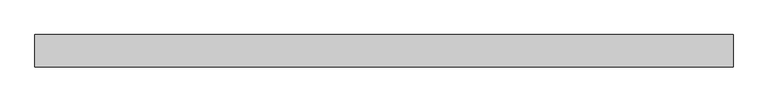
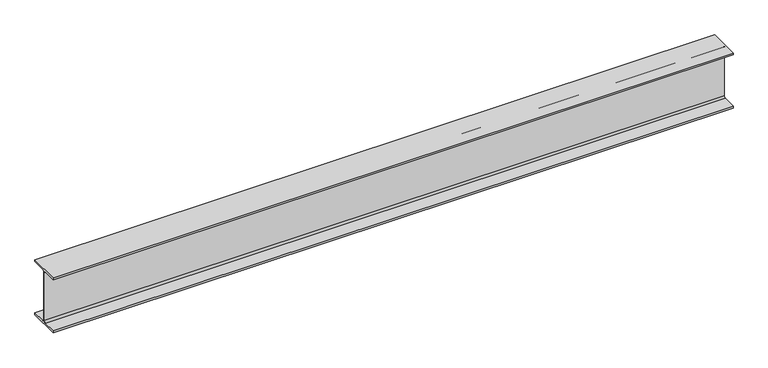
"""IFC4 building model written with IfcOpenShell, lengths in millimetres: beam geometry, Steel Beam_H-KSD3502 : H_SB_ASB_H-200x200x8x12."""

import ifcopenshell
import ifcopenshell.guid

model = None  # the IFC model being written
_history = None  # IfcOwnerHistory: only IFC2X3 demands one
_inside = {}  # id of a spatial element -> (the spatial element, [elements in it])
_under = {}  # id of a project, library or spatial element -> (it, [spatial elements below it])
_declared = {}  # id of a project -> (the project, [libraries it declares])
_typed = {}  # id of a type object -> (the type object, [elements of that type])
_made_of = {}  # id of a material, layer set ... -> (it, [elements and type objects made of it])


def new_model(schema):
    """Start an empty IFC model of exactly this schema.

    Asked for "IFC4X3", IfcOpenShell would pick the latest addendum, in which some entities
    have other attributes; the version numbers below select the first issue.
    IFC2X3 requires an IfcOwnerHistory on every rooted entity: one is made here for all.
    """
    global model, _history
    if schema == "IFC4X3":
        model = ifcopenshell.file(schema_version=(4, 3, 0, 0))
    else:
        model = ifcopenshell.file(schema=schema)
    _inside.clear()
    _under.clear()
    _declared.clear()
    _typed.clear()
    _made_of.clear()
    _history = None
    if model.schema == "IFC2X3":
        org = make("IfcOrganization", Name="unknown")
        user = make(
            "IfcPersonAndOrganization",
            ThePerson=make("IfcPerson", FamilyName="unknown"),
            TheOrganization=org,
        )
        app = make(
            "IfcApplication",
            ApplicationDeveloper=org,
            Version="unknown",
            ApplicationFullName="unknown",
            ApplicationIdentifier="unknown",
        )
        _history = make(
            "IfcOwnerHistory",
            OwningUser=user,
            OwningApplication=app,
            ChangeAction="ADDED",
            CreationDate=0,
        )
    return model


def make(cls, **values):
    """One entity of the class cls with the attributes given. An attribute that is None is left unset."""
    return model.create_entity(
        cls, **{name: value for name, value in values.items() if value is not None}
    )


def rooted(cls, **values):
    """An entity with a GlobalId (a new one), such as an element, a storey or a relation."""
    return make(cls, GlobalId=ifcopenshell.guid.new(), OwnerHistory=_history, **values)


def si_unit(unit_type, name, prefix=None):
    """IfcSIUnit, for example si_unit("LENGTHUNIT", "METRE", prefix="MILLI")."""
    return make("IfcSIUnit", UnitType=unit_type, Prefix=prefix, Name=name)


def assignment(units):
    """IfcUnitAssignment: the units of a project."""
    return None if units is None else make("IfcUnitAssignment", Units=units)


def point(xyz):
    """IfcCartesianPoint."""
    return None if xyz is None else make("IfcCartesianPoint", Coordinates=xyz)


def direction(xyz):
    """IfcDirection."""
    return None if xyz is None else make("IfcDirection", DirectionRatios=xyz)


def frame(location, z_axis=None, x_axis=None):
    """IfcAxis2Placement3D, a coordinate frame: its origin and axes. An axis left out is left unset."""
    return make(
        "IfcAxis2Placement3D",
        Location=point(location),
        Axis=direction(z_axis),
        RefDirection=direction(x_axis),
    )


def frame_2d(location, x_axis=None):
    """IfcAxis2Placement2D, a coordinate frame in the plane: its origin and x axis."""
    return make(
        "IfcAxis2Placement2D", Location=point(location), RefDirection=direction(x_axis)
    )


def origin():
    """The frame at (0, 0, 0) with its axes left unset."""
    return frame((0.0, 0.0, 0.0))


def place(relative_to, where):
    """IfcLocalPlacement: puts the frame where relative to a parent placement (None: the world)."""
    return make(
        "IfcLocalPlacement", PlacementRelTo=relative_to, RelativePlacement=where
    )


def context(
    kind, dimensions, precision=None, world=None, true_north=None, identifier=None
):
    """IfcGeometricRepresentationContext, for example the 3D "Model" context."""
    return make(
        "IfcGeometricRepresentationContext",
        ContextIdentifier=identifier,
        ContextType=kind,
        CoordinateSpaceDimension=dimensions,
        Precision=precision,
        WorldCoordinateSystem=world,
        TrueNorth=true_north,
    )


def project(units=None, contexts=None):
    """IfcProject with its units and contexts."""
    return rooted(
        "IfcProject",
        Name="project",
        RepresentationContexts=contexts,
        UnitsInContext=assignment(units),
    )


def spatial(cls, under=None, at=None, **own):
    """A site, building, storey or space (cls), placed at a placement, below another one or the project."""
    s = rooted(cls, ObjectPlacement=at, **own)
    if under is not None:
        _under.setdefault(under.id(), (under, []))[1].append(s)
    return s


def polyline(points):
    """IfcPolyline through the points."""
    return make("IfcPolyline", Points=[point(p) for p in points])


def circle_curve(where, radius):
    """IfcCircle in the frame where."""
    return make("IfcCircle", Position=where, Radius=radius)


def trimmed(basis, trim1, trim2, sense, master):
    """IfcTrimmedCurve: the piece of a basis curve between two trims."""
    return make(
        "IfcTrimmedCurve",
        BasisCurve=basis,
        Trim1=trim1,
        Trim2=trim2,
        SenseAgreement=sense,
        MasterRepresentation=master,
    )


def segment(curve, same_sense, transition):
    """IfcCompositeCurveSegment."""
    return make(
        "IfcCompositeCurveSegment",
        Transition=transition,
        SameSense=same_sense,
        ParentCurve=curve,
    )


def composite_curve(segments, self_intersect=None):
    """IfcCompositeCurve: segments joined end to end."""
    return make("IfcCompositeCurve", Segments=segments, SelfIntersect=self_intersect)


def outline(outer, holes=None, kind="AREA"):
    """IfcArbitraryClosedProfileDef: a profile drawn as a closed curve; with holes, ...WithVoids."""
    if holes is None:
        return make("IfcArbitraryClosedProfileDef", ProfileType=kind, OuterCurve=outer)
    return make(
        "IfcArbitraryProfileDefWithVoids",
        ProfileType=kind,
        OuterCurve=outer,
        InnerCurves=holes,
    )


def extrude(swept, where, along, depth):
    """IfcExtrudedAreaSolid: the profile swept, set in the frame where, extruded along a direction by depth."""
    return make(
        "IfcExtrudedAreaSolid",
        SweptArea=swept,
        Position=where,
        ExtrudedDirection=direction(along),
        Depth=depth,
    )


def shape(context_of_items, identifier, shape_type, items):
    """IfcShapeRepresentation: the items that make up one representation, for example the "Body"."""
    return make(
        "IfcShapeRepresentation",
        ContextOfItems=context_of_items,
        RepresentationIdentifier=identifier,
        RepresentationType=shape_type,
        Items=items,
    )


def source(mapping_origin, context_of_items, identifier, shape_type, items):
    """IfcRepresentationMap: a shape defined once, which mapped items show again and again."""
    return make(
        "IfcRepresentationMap",
        MappingOrigin=mapping_origin,
        MappedRepresentation=shape(context_of_items, identifier, shape_type, items),
    )


def transform(
    local_origin,
    x_axis=None,
    y_axis=None,
    z_axis=None,
    scale=None,
    scale2=None,
    scale3=None,
    uniform=True,
):
    """IfcCartesianTransformationOperator3D, or its non-uniform kind. x_axis, y_axis, z_axis: its Axis1, 2, 3."""
    if uniform:
        return make(
            "IfcCartesianTransformationOperator3D",
            Axis1=direction(x_axis),
            Axis2=direction(y_axis),
            LocalOrigin=point(local_origin),
            Scale=scale,
            Axis3=direction(z_axis),
        )
    return make(
        "IfcCartesianTransformationOperator3DnonUniform",
        Axis1=direction(x_axis),
        Axis2=direction(y_axis),
        LocalOrigin=point(local_origin),
        Scale=scale,
        Axis3=direction(z_axis),
        Scale2=scale2,
        Scale3=scale3,
    )


def mapped(mapping_source, mapping_target):
    """IfcMappedItem: shows the shape of a source again, moved by a transform."""
    return make(
        "IfcMappedItem", MappingSource=mapping_source, MappingTarget=mapping_target
    )


def made_of(thing, what):
    """Note that an element or type object is made of a material, layer set ...; save() writes the relation."""
    if what is not None:
        _made_of.setdefault(what.id(), (what, []))[1].append(thing)
    return thing


def element(
    cls,
    number,
    at=None,
    inside=None,
    cuts=None,
    type_object=None,
    material=None,
    context=None,
    identifier="Body",
    shape_type=None,
    held_by="IfcProductDefinitionShape",
    body=None,
    shapes=None,
    **own,
):
    """One element of the class cls, such as IfcWall. Its Tag is "e" and its number.

    at: its placement. inside: the storey or other place that contains it. cuts: it is an
    opening in that element (IfcRelVoidsElement). A single representation is given by context,
    identifier, shape_type and body (its items); several are given by shapes. held_by: the class
    of the entity that holds the representations. save() writes the other relations.
    """
    e = rooted(cls, Tag="e%d" % number, ObjectPlacement=at, **own)
    if body is not None:
        shapes = [shape(context, identifier, shape_type, body)]
    if shapes is not None:
        e.Representation = make(held_by, Representations=shapes)
    if inside is not None:
        _inside.setdefault(inside.id(), (inside, []))[1].append(e)
    if cuts is not None:
        rooted(
            "IfcRelVoidsElement", RelatingBuildingElement=cuts, RelatedOpeningElement=e
        )
    if type_object is not None:
        _typed.setdefault(type_object.id(), (type_object, []))[1].append(e)
    return made_of(e, material)


def aggregate(whole, parts):
    """IfcRelAggregates: a whole, such as a stair, and the parts it consists of."""
    return rooted("IfcRelAggregates", RelatingObject=whole, RelatedObjects=parts)


def save(model, path):
    """Write the relations noted so far, then the file.

    IfcRelAggregates (storeys below a building ...), IfcRelContainedInSpatialStructure (elements
    in a storey), IfcRelDefinesByType, IfcRelAssociatesMaterial and IfcRelDeclares: one each for
    every whole, place, type object, material and project.
    """
    for whole, parts in _under.values():
        aggregate(whole, parts)
    for where, things in _inside.values():
        rooted(
            "IfcRelContainedInSpatialStructure",
            RelatedElements=things,
            RelatingStructure=where,
        )
    for kind, things in _typed.values():
        rooted("IfcRelDefinesByType", RelatedObjects=things, RelatingType=kind)
    for what, things in _made_of.values():
        rooted("IfcRelAssociatesMaterial", RelatedObjects=things, RelatingMaterial=what)
    for by, libraries in _declared.values():
        rooted("IfcRelDeclares", RelatingContext=by, RelatedDefinitions=libraries)
    model.write(path)


def beam_b41741f2(model_context):
    return source(origin(), model_context, "Body", "SweptSolid", [
        extrude(outline(composite_curve([segment(polyline([(82.5, -141.5), (82.5, -151.7), (-82.5, -151.7), (-82.5, -141.5), (-11.9, -141.5)]), True, "CONTINUOUS"), segment(trimmed(circle_curve(frame_2d((-11.9, -132.6)), 8.9), [point((-11.9, -141.5))], [point((-3.0, -132.6))], True, "CARTESIAN"), True, "CONTINUOUS"), segment(polyline([(-3.0, -132.6), (-3.0, 132.6)]), True, "CONTINUOUS"), segment(trimmed(circle_curve(frame_2d((-11.9, 132.6)), 8.9), [point((-3.0, 132.6))], [point((-11.9, 141.5))], True, "CARTESIAN"), True, "CONTINUOUS"), segment(polyline([(-11.9, 141.5), (-82.5, 141.5), (-82.5, 151.7), (82.5, 151.7), (82.5, 141.5), (11.9, 141.5)]), True, "CONTINUOUS"), segment(trimmed(circle_curve(frame_2d((11.9, 132.6)), 8.9), [point((11.9, 141.5))], [point((3.0, 132.6))], True, "CARTESIAN"), True, "CONTINUOUS"), segment(polyline([(3.0, 132.6), (3.0, -132.6)]), True, "CONTINUOUS"), segment(trimmed(circle_curve(frame_2d((11.9, -132.6)), 8.9), [point((3.0, -132.6))], [point((11.9, -141.5))], True, "CARTESIAN"), True, "CONTINUOUS"), segment(polyline([(11.9, -141.5), (82.5, -141.5)]), True, "CONTINUOUS")], self_intersect=False)), frame((-1826.0344939, 0.0, 0.0), z_axis=(1.0, 0.0, 0.0), x_axis=(0.0, 1.0, 0.0)), (0.0, 0.0, 1.0), 3548.8457304),
    ])


if __name__ == "__main__":
    model = new_model("IFC4")
    model_context = context("Model", 3, world=origin())
    ifc_project = project(units=[si_unit("LENGTHUNIT", "METRE", prefix="MILLI")], contexts=[model_context])
    site = spatial("IfcSite", under=ifc_project)
    building = spatial("IfcBuilding", under=site)
    placement = place(None, origin())
    beam_shape = beam_b41741f2(model_context)
    element("IfcBeam", 1, ObjectType="Steel Beam_H-KSD3502 : H_SB_ASB_H-200x200x8x12", at=placement, inside=building, context=model_context, shape_type="MappedRepresentation", body=[
        mapped(beam_shape, transform((0.0, 0.0, 0.0), x_axis=(1.0, 0.0, 0.0), y_axis=(0.0, 1.0, 0.0), z_axis=(0.0, 0.0, 1.0))),
    ])
    save(model, "model.ifc")

# Revit data of these elements
# Type "Steel Beam_H-KSD3502 : H_SB_ASB_H-200x200x8x12"
#   Width = 20.0 cm
#   Web Thickness = 0.8 cm
#   Web Fillet = 1.3 cm
#   Warping Constant = 141376.0 cm⁶
#   Torsional Moment of Inertia = 26.2485 cm⁴
#   Torsional Modulus = 1.0 cm³
#   Section Area = 63.53 cm²
#   Plastic Modulus weak axis = 244.0 cm³
#   Plastic Modulus strong axis = 525.0 cm³
#   Perimeter = 1.16 m²/m
#   Nominal Weight = 49.90 kgf/m
#   Moment of Inertia weak axis = 1600.00 cm⁴
#   Moment of Inertia strong axis = 4720.00 cm⁴
#   Height = 20.0 cm
#   Flange Thickness = 1.2 cm
#   Elastic Modulus weak axis = 160.0 cm³
#   Elastic Modulus strong axis = 472.0 cm³
#   Centroid Vertical = 10.0 cm
#   Centroid Horizontal = 10.0 cm
#   Length [instance default] = 1.5240 m
#   Structural Material [instance default] = Steel, 45-345
#   Assembly Code = ""
# Element 1 (IfcBeam, "Steel Beam_H-KSD3502 : H_SB_ASB_H-200x200x8x12")
#   Structural Material = none
# Materials
#   "Steel, 45-345": class "Metal", colour RGB 189 187 185, transparency 0, Description = "Steel 345 MPa", Cost = 0
